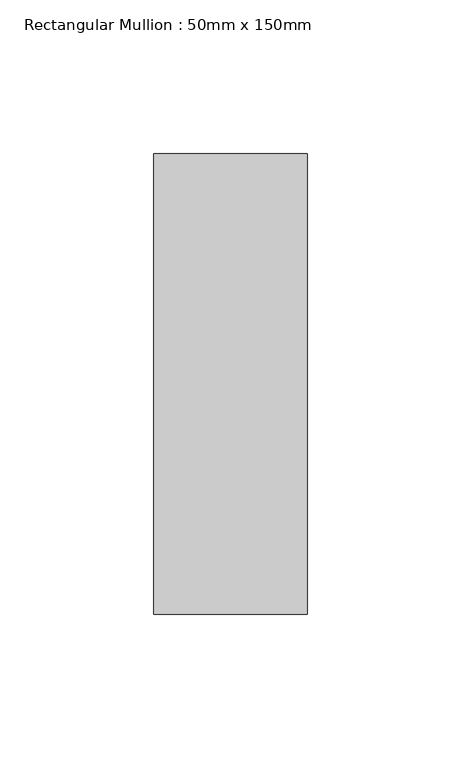
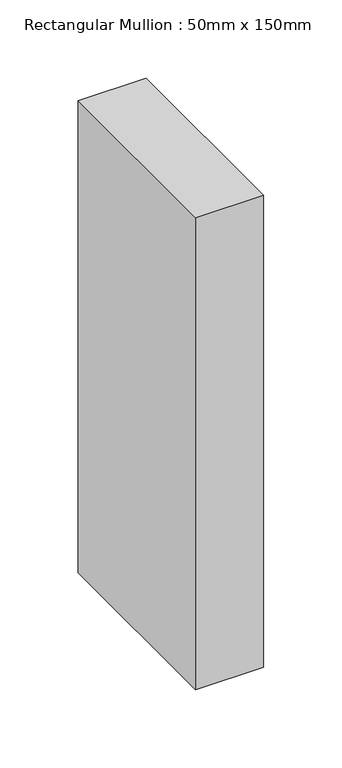
"""IFC4 building model written with IfcOpenShell, lengths in millimetres: member geometry, Rectangular Mullion : 50mm x 150mm."""

from ifc_helpers import new_model, si_unit, frame, origin, place, context, project, spatial, polyline, outline, extrude, source, transform, mapped, element, save


def rectangular_mullion_50mm_x_150mm_d9aeadd2(model_context):
    return source(origin(), model_context, "Body", "SweptSolid", [
        extrude(outline(polyline([(0.0, 75.0), (0.0, -75.0), (-50.0, -75.0), (-50.0, 75.0), (0.0, 75.0)])), frame((0.0, 0.0, -367.6767677), z_axis=(0.0, 0.0, 1.0), x_axis=(1.0, 0.0, 0.0)), (0.0, 0.0, 1.0), 367.6767677),
    ])


if __name__ == "__main__":
    model = new_model("IFC4")
    model_context = context("Model", 3, world=origin())
    ifc_project = project(units=[si_unit("LENGTHUNIT", "METRE", prefix="MILLI")], contexts=[model_context])
    site = spatial("IfcSite", under=ifc_project)
    building = spatial("IfcBuilding", under=site)
    placement = place(None, origin())
    rectangular_mullion_50mm_x_150mm_shape = rectangular_mullion_50mm_x_150mm_d9aeadd2(model_context)
    element("IfcMember", 1, ObjectType="Rectangular Mullion : 50mm x 150mm", at=placement, inside=building, context=model_context, shape_type="MappedRepresentation", body=[
        mapped(rectangular_mullion_50mm_x_150mm_shape, transform((0.0, 0.0, 0.0), x_axis=(1.0, 0.0, 0.0), y_axis=(0.0, 1.0, 0.0), z_axis=(0.0, 0.0, 1.0))),
    ])
    save(model, "model.ifc")

# Revit data of these elements
# Type "Rectangular Mullion : 50mm x 150mm"
#   built-in parameter 1007304 = 0.492126 (stored number, unit not read)
#   built-in parameter 1007301 = 0.082021 (stored number, unit not read)
#   built-in parameter 1007300 = 0.082021 (stored number, unit not read)
# Element 1 (IfcMember, "Rectangular Mullion : 50mm x 150mm")
#   Materials on its faces: "Aluminum"
# Materials
#   "Aluminum": class "Metal", colour RGB 244 244 244, transparency 0, Description = "Aluminum 6061", Cost = 0
